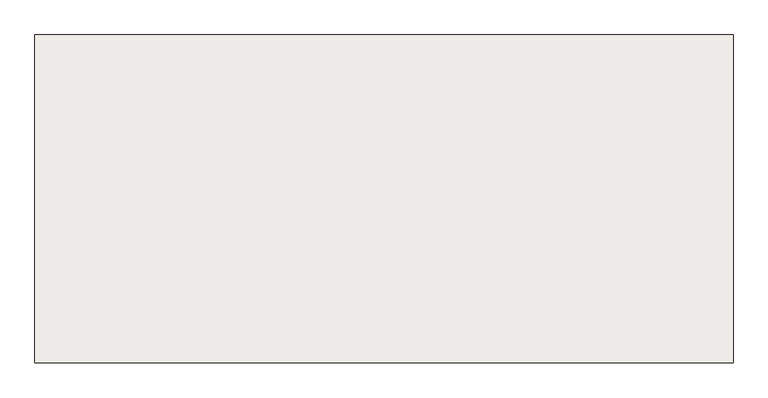
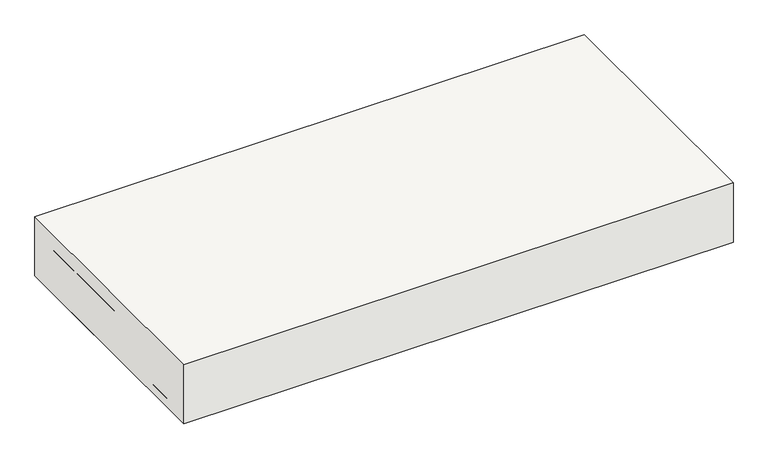
"""IFC4 building model written with IfcOpenShell, lengths in millimetres: slab geometry, Pano 21 (16 cm)."""

import ifcopenshell
import ifcopenshell.guid

model = None  # the IFC model being written
_history = None  # IfcOwnerHistory: only IFC2X3 demands one
_inside = {}  # id of a spatial element -> (the spatial element, [elements in it])
_under = {}  # id of a project, library or spatial element -> (it, [spatial elements below it])
_declared = {}  # id of a project -> (the project, [libraries it declares])
_typed = {}  # id of a type object -> (the type object, [elements of that type])
_made_of = {}  # id of a material, layer set ... -> (it, [elements and type objects made of it])


def new_model(schema):
    """Start an empty IFC model of exactly this schema.

    Asked for "IFC4X3", IfcOpenShell would pick the latest addendum, in which some entities
    have other attributes; the version numbers below select the first issue.
    IFC2X3 requires an IfcOwnerHistory on every rooted entity: one is made here for all.
    """
    global model, _history
    if schema == "IFC4X3":
        model = ifcopenshell.file(schema_version=(4, 3, 0, 0))
    else:
        model = ifcopenshell.file(schema=schema)
    _inside.clear()
    _under.clear()
    _declared.clear()
    _typed.clear()
    _made_of.clear()
    _history = None
    if model.schema == "IFC2X3":
        org = make("IfcOrganization", Name="unknown")
        user = make(
            "IfcPersonAndOrganization",
            ThePerson=make("IfcPerson", FamilyName="unknown"),
            TheOrganization=org,
        )
        app = make(
            "IfcApplication",
            ApplicationDeveloper=org,
            Version="unknown",
            ApplicationFullName="unknown",
            ApplicationIdentifier="unknown",
        )
        _history = make(
            "IfcOwnerHistory",
            OwningUser=user,
            OwningApplication=app,
            ChangeAction="ADDED",
            CreationDate=0,
        )
    return model


def make(cls, **values):
    """One entity of the class cls with the attributes given. An attribute that is None is left unset."""
    return model.create_entity(
        cls, **{name: value for name, value in values.items() if value is not None}
    )


def rooted(cls, **values):
    """An entity with a GlobalId (a new one), such as an element, a storey or a relation."""
    return make(cls, GlobalId=ifcopenshell.guid.new(), OwnerHistory=_history, **values)


def si_unit(unit_type, name, prefix=None):
    """IfcSIUnit, for example si_unit("LENGTHUNIT", "METRE", prefix="MILLI")."""
    return make("IfcSIUnit", UnitType=unit_type, Prefix=prefix, Name=name)


def assignment(units):
    """IfcUnitAssignment: the units of a project."""
    return None if units is None else make("IfcUnitAssignment", Units=units)


def point(xyz):
    """IfcCartesianPoint."""
    return None if xyz is None else make("IfcCartesianPoint", Coordinates=xyz)


def direction(xyz):
    """IfcDirection."""
    return None if xyz is None else make("IfcDirection", DirectionRatios=xyz)


def frame(location, z_axis=None, x_axis=None):
    """IfcAxis2Placement3D, a coordinate frame: its origin and axes. An axis left out is left unset."""
    return make(
        "IfcAxis2Placement3D",
        Location=point(location),
        Axis=direction(z_axis),
        RefDirection=direction(x_axis),
    )


def origin():
    """The frame at (0, 0, 0) with its axes left unset."""
    return frame((0.0, 0.0, 0.0))


def origin_with_axes():
    """The frame at (0, 0, 0) with the z axis (0, 0, 1) and the x axis (1, 0, 0) written out."""
    return frame((0.0, 0.0, 0.0), z_axis=(0.0, 0.0, 1.0), x_axis=(1.0, 0.0, 0.0))


def place(relative_to, where):
    """IfcLocalPlacement: puts the frame where relative to a parent placement (None: the world)."""
    return make(
        "IfcLocalPlacement", PlacementRelTo=relative_to, RelativePlacement=where
    )


def context(
    kind, dimensions, precision=None, world=None, true_north=None, identifier=None
):
    """IfcGeometricRepresentationContext, for example the 3D "Model" context."""
    return make(
        "IfcGeometricRepresentationContext",
        ContextIdentifier=identifier,
        ContextType=kind,
        CoordinateSpaceDimension=dimensions,
        Precision=precision,
        WorldCoordinateSystem=world,
        TrueNorth=true_north,
    )


def project(units=None, contexts=None):
    """IfcProject with its units and contexts."""
    return rooted(
        "IfcProject",
        Name="project",
        RepresentationContexts=contexts,
        UnitsInContext=assignment(units),
    )


def spatial(cls, under=None, at=None, **own):
    """A site, building, storey or space (cls), placed at a placement, below another one or the project."""
    s = rooted(cls, ObjectPlacement=at, **own)
    if under is not None:
        _under.setdefault(under.id(), (under, []))[1].append(s)
    return s


def polyline(points):
    """IfcPolyline through the points."""
    return make("IfcPolyline", Points=[point(p) for p in points])


def outline(outer, holes=None, kind="AREA"):
    """IfcArbitraryClosedProfileDef: a profile drawn as a closed curve; with holes, ...WithVoids."""
    if holes is None:
        return make("IfcArbitraryClosedProfileDef", ProfileType=kind, OuterCurve=outer)
    return make(
        "IfcArbitraryProfileDefWithVoids",
        ProfileType=kind,
        OuterCurve=outer,
        InnerCurves=holes,
    )


def extrude(swept, where, along, depth):
    """IfcExtrudedAreaSolid: the profile swept, set in the frame where, extruded along a direction by depth."""
    return make(
        "IfcExtrudedAreaSolid",
        SweptArea=swept,
        Position=where,
        ExtrudedDirection=direction(along),
        Depth=depth,
    )


def shape(context_of_items, identifier, shape_type, items):
    """IfcShapeRepresentation: the items that make up one representation, for example the "Body"."""
    return make(
        "IfcShapeRepresentation",
        ContextOfItems=context_of_items,
        RepresentationIdentifier=identifier,
        RepresentationType=shape_type,
        Items=items,
    )


def source(mapping_origin, context_of_items, identifier, shape_type, items):
    """IfcRepresentationMap: a shape defined once, which mapped items show again and again."""
    return make(
        "IfcRepresentationMap",
        MappingOrigin=mapping_origin,
        MappedRepresentation=shape(context_of_items, identifier, shape_type, items),
    )


def transform(
    local_origin,
    x_axis=None,
    y_axis=None,
    z_axis=None,
    scale=None,
    scale2=None,
    scale3=None,
    uniform=True,
):
    """IfcCartesianTransformationOperator3D, or its non-uniform kind. x_axis, y_axis, z_axis: its Axis1, 2, 3."""
    if uniform:
        return make(
            "IfcCartesianTransformationOperator3D",
            Axis1=direction(x_axis),
            Axis2=direction(y_axis),
            LocalOrigin=point(local_origin),
            Scale=scale,
            Axis3=direction(z_axis),
        )
    return make(
        "IfcCartesianTransformationOperator3DnonUniform",
        Axis1=direction(x_axis),
        Axis2=direction(y_axis),
        LocalOrigin=point(local_origin),
        Scale=scale,
        Axis3=direction(z_axis),
        Scale2=scale2,
        Scale3=scale3,
    )


def mapped(mapping_source, mapping_target):
    """IfcMappedItem: shows the shape of a source again, moved by a transform."""
    return make(
        "IfcMappedItem", MappingSource=mapping_source, MappingTarget=mapping_target
    )


def made_of(thing, what):
    """Note that an element or type object is made of a material, layer set ...; save() writes the relation."""
    if what is not None:
        _made_of.setdefault(what.id(), (what, []))[1].append(thing)
    return thing


def element(
    cls,
    number,
    at=None,
    inside=None,
    cuts=None,
    type_object=None,
    material=None,
    context=None,
    identifier="Body",
    shape_type=None,
    held_by="IfcProductDefinitionShape",
    body=None,
    shapes=None,
    **own,
):
    """One element of the class cls, such as IfcWall. Its Tag is "e" and its number.

    at: its placement. inside: the storey or other place that contains it. cuts: it is an
    opening in that element (IfcRelVoidsElement). A single representation is given by context,
    identifier, shape_type and body (its items); several are given by shapes. held_by: the class
    of the entity that holds the representations. save() writes the other relations.
    """
    e = rooted(cls, Tag="e%d" % number, ObjectPlacement=at, **own)
    if body is not None:
        shapes = [shape(context, identifier, shape_type, body)]
    if shapes is not None:
        e.Representation = make(held_by, Representations=shapes)
    if inside is not None:
        _inside.setdefault(inside.id(), (inside, []))[1].append(e)
    if cuts is not None:
        rooted(
            "IfcRelVoidsElement", RelatingBuildingElement=cuts, RelatedOpeningElement=e
        )
    if type_object is not None:
        _typed.setdefault(type_object.id(), (type_object, []))[1].append(e)
    return made_of(e, material)


def aggregate(whole, parts):
    """IfcRelAggregates: a whole, such as a stair, and the parts it consists of."""
    return rooted("IfcRelAggregates", RelatingObject=whole, RelatedObjects=parts)


def save(model, path):
    """Write the relations noted so far, then the file.

    IfcRelAggregates (storeys below a building ...), IfcRelContainedInSpatialStructure (elements
    in a storey), IfcRelDefinesByType, IfcRelAssociatesMaterial and IfcRelDeclares: one each for
    every whole, place, type object, material and project.
    """
    for whole, parts in _under.values():
        aggregate(whole, parts)
    for where, things in _inside.values():
        rooted(
            "IfcRelContainedInSpatialStructure",
            RelatedElements=things,
            RelatingStructure=where,
        )
    for kind, things in _typed.values():
        rooted("IfcRelDefinesByType", RelatedObjects=things, RelatingType=kind)
    for what, things in _made_of.values():
        rooted("IfcRelAssociatesMaterial", RelatedObjects=things, RelatingMaterial=what)
    for by, libraries in _declared.values():
        rooted("IfcRelDeclares", RelatingContext=by, RelatedDefinitions=libraries)
    model.write(path)


def slab_03f20a11(model_context):
    return source(origin(), model_context, "Body", "SweptSolid", [
        extrude(outline(polyline([(3800.0, 11155.0), (3800.0, 10495.0), (2395.00107, 10495.0), (2395.00107, 11155.0), (3800.0, 11155.0)])), origin_with_axes(), (0.0, 0.0, 1.0), 160.0),
        extrude(outline(polyline([(3395.00107, 10710.5), (3395.00107, 11070.5), (3795.0, 11070.5), (3795.0, 10710.5), (3395.00107, 10710.5)])), origin_with_axes(), (0.0, 0.0, 1.0), 120.0),
        extrude(outline(polyline([(2895.00107, 10710.5), (2895.00107, 11070.5), (3390.00107, 11070.5), (3390.00107, 10710.5), (2895.00107, 10710.5)])), origin_with_axes(), (0.0, 0.0, 1.0), 120.0),
        extrude(outline(polyline([(2395.00107, 10571.0), (2395.00107, 10711.0), (3800.0, 10711.0), (3800.0, 10571.0), (2395.00107, 10571.0)])), origin_with_axes(), (0.0, 0.0, 1.0), 24.0),
        extrude(outline(polyline([(2395.00107, 10710.5), (2395.00107, 11070.5), (2890.00107, 11070.5), (2890.00107, 10710.5), (2395.00107, 10710.5)])), origin_with_axes(), (0.0, 0.0, 1.0), 120.0),
    ])


if __name__ == "__main__":
    model = new_model("IFC4")
    model_context = context("Model", 3, world=origin())
    ifc_project = project(units=[si_unit("LENGTHUNIT", "METRE", prefix="MILLI")], contexts=[model_context])
    site = spatial("IfcSite", under=ifc_project)
    building = spatial("IfcBuilding", under=site)
    placement = place(None, origin())
    slab_shape = slab_03f20a11(model_context)
    element("IfcSlab", 1, ObjectType="Pano 21 (16 cm)", at=placement, inside=building, context=model_context, shape_type="MappedRepresentation", body=[
        mapped(slab_shape, transform((0.0, 0.0, 0.0), x_axis=(1.0, 0.0, 0.0), y_axis=(0.0, 1.0, 0.0), z_axis=(0.0, 0.0, 1.0))),
    ])
    save(model, "model.ifc")

# Revit data of these elements
# Project information
#   Autor = "Rafael Bragagnolo Lima"
#   Data de emissão do projeto = "Data de emissão"
#   Status do projeto = "Status do projeto"
#   Nome do cliente = "RR Engenharia"
#   Endereço do projeto = "São Paulo - SP"
#   Nome do projeto = "Revit Estrutural 2024"
#   Número do projeto = "Número do projeto"
# Element 1 (IfcSlab, "Pano 21 (16 cm)")
#   Materials on its faces: "Molde de poliestireno", "RGB 168-169-158", "Concreto armado"
# Materials
#   "Molde de poliestireno": class "Não atribuído", colour RGB 255 255 255, transparency 0
#   "RGB 168-169-158": class "Não atribuído", colour RGB 168 169 158, transparency 0
#   "Concreto armado": class "Não atribuído", colour RGB 168 169 158, transparency 0
